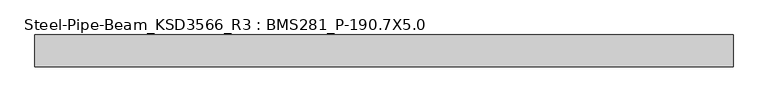
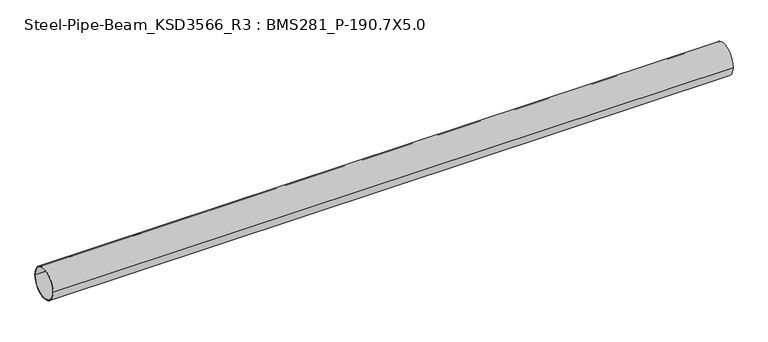
"""IFC4 building model written with IfcOpenShell, lengths in millimetres: member geometry, Steel-Pipe-Beam_KSD3566_R3 : BMS281_P-190.7X5.0."""

from ifc_helpers import new_model, si_unit, point, frame, origin, origin_2d, place, context, project, spatial, circle_curve, trimmed, segment, composite_curve, outline, extrude, source, transform, mapped, element, save


def steel_pipe_beam_ksd3566_r3_bms281_p_190_7x5_0_91d91e60(model_context):
    return source(origin(), model_context, "Body", "SweptSolid", [
        extrude(outline(composite_curve([segment(trimmed(circle_curve(origin_2d(), 95.35), [point((-95.35, 0.0))], [point((95.35, 0.0))], False, "CARTESIAN"), True, "CONTINUOUS"), segment(trimmed(circle_curve(origin_2d(), 95.35), [point((95.35, 0.0))], [point((-95.35, 0.0))], False, "CARTESIAN"), True, "CONTINUOUS")], self_intersect=False), holes=[composite_curve([segment(trimmed(circle_curve(origin_2d(), 90.35), [point((90.35, 0.0))], [point((-90.35, 0.0))], True, "CARTESIAN"), True, "CONTINUOUS"), segment(trimmed(circle_curve(origin_2d(), 90.35), [point((-90.35, 0.0))], [point((90.35, 0.0))], True, "CARTESIAN"), True, "CONTINUOUS")], self_intersect=False)]), frame((-2059.528929, 0.0, 0.0), z_axis=(1.0, 0.0, 0.0), x_axis=(0.0, 1.0, 0.0)), (0.0, 0.0, 1.0), 4153.3992791),
    ])


if __name__ == "__main__":
    model = new_model("IFC4")
    model_context = context("Model", 3, world=origin())
    ifc_project = project(units=[si_unit("LENGTHUNIT", "METRE", prefix="MILLI")], contexts=[model_context])
    site = spatial("IfcSite", under=ifc_project)
    building = spatial("IfcBuilding", under=site)
    placement = place(None, origin())
    steel_pipe_beam_ksd3566_r3_bms281_p_190_7x5_0_shape = steel_pipe_beam_ksd3566_r3_bms281_p_190_7x5_0_91d91e60(model_context)
    element("IfcMember", 1, ObjectType="Steel-Pipe-Beam_KSD3566_R3 : BMS281_P-190.7X5.0", at=placement, inside=building, context=model_context, shape_type="MappedRepresentation", body=[
        mapped(steel_pipe_beam_ksd3566_r3_bms281_p_190_7x5_0_shape, transform((0.0, 0.0, 0.0), x_axis=(1.0, 0.0, 0.0), y_axis=(0.0, 1.0, 0.0), z_axis=(0.0, 0.0, 1.0))),
    ])
    save(model, "model.ifc")

# Revit data of these elements
# Type "Steel-Pipe-Beam_KSD3566_R3 : BMS281_P-190.7X5.0"
#   Keynote = "P-190.7X5.0"
#   SteelWeight = "Light"
#   t = 0.0050 m
#   Surface Area = 0.599102 m²/m
#   Section Area = 29.1697 cm²
#   Mass per Unit Length = 22.8982 kg/m
#   Length [instance default] = 1.5000 m
#   D = 0.1907 m
#   hec_material4 [instance default] = none
#   hec_material3 [instance default] = none
#   hec_material2 [instance default] = none
#   hec_material1 [instance default] = none
#   Structural Material [instance default] = Steel, 45-345
#   Assembly Code = ""
# Element 1 (IfcMember, "Steel-Pipe-Beam_KSD3566_R3 : BMS281_P-190.7X5.0")
#   Structural Material = none
# Materials
#   "Steel, 45-345": class "Metal", colour RGB 189 187 185, transparency 0, Description = "Steel 345 MPa", Cost = 0
